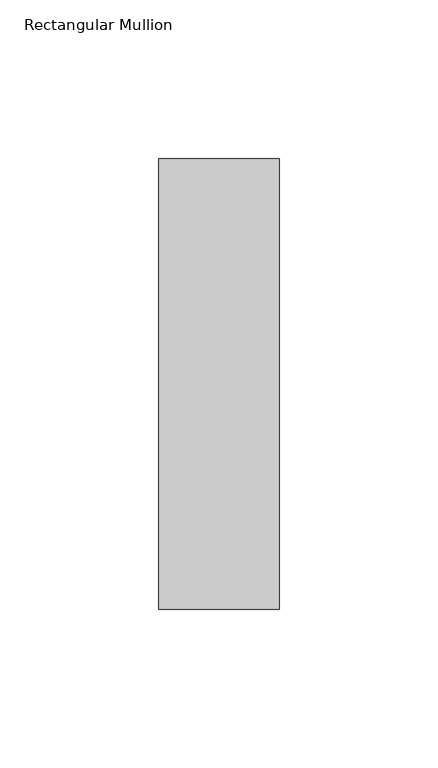
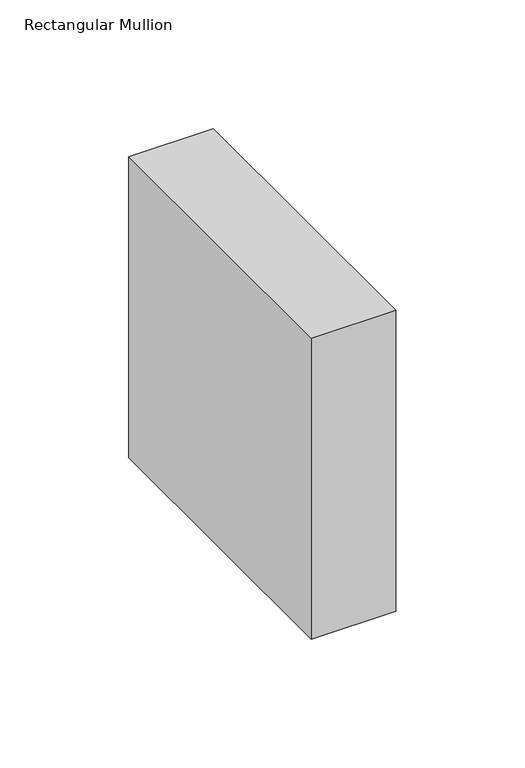
"""IFC4 building model written with IfcOpenShell, lengths in millimetres: member geometry, Rectangular Mullion : NLRS_21_CWM_hsb-regel 38x142_gen_rsf."""

from ifc_helpers import new_model, si_unit, frame, origin, place, context, project, spatial, polyline, outline, extrude, source, transform, mapped, element, save


def rectangular_mullion_f3eb0596(model_context):
    return source(origin(), model_context, "Body", "SweptSolid", [
        extrude(outline(polyline([(0.0, -71.0), (-38.0, -71.0), (-38.0, 71.0), (0.0, 71.0), (0.0, -71.0)])), frame((0.0, 0.0, -142.9999997), z_axis=(0.0, 0.0, 1.0), x_axis=(1.0, 0.0, 0.0)), (0.0, 0.0, 1.0), 142.9999997),
    ])


if __name__ == "__main__":
    model = new_model("IFC4")
    model_context = context("Model", 3, world=origin())
    ifc_project = project(units=[si_unit("LENGTHUNIT", "METRE", prefix="MILLI")], contexts=[model_context])
    site = spatial("IfcSite", under=ifc_project)
    building = spatial("IfcBuilding", under=site)
    placement = place(None, origin())
    rectangular_mullion_shape = rectangular_mullion_f3eb0596(model_context)
    element("IfcMember", 1, ObjectType="Rectangular Mullion : NLRS_21_CWM_hsb-regel 38x142_gen_rsf", at=placement, inside=building, context=model_context, shape_type="MappedRepresentation", body=[
        mapped(rectangular_mullion_shape, transform((0.0, 0.0, 0.0), x_axis=(1.0, 0.0, 0.0), y_axis=(0.0, 1.0, 0.0), z_axis=(0.0, 0.0, 1.0))),
    ])
    save(model, "model.ifc")

# Revit data of these elements
# Type "Rectangular Mullion : NLRS_21_CWM_hsb-regel 38x142_gen_rsf"
#   Export Type to IFC As = "IfcWall"
#   Type IfcGUID = "07M7mRoiH1CR8m_RSKIwpF"
#   Assembly Code = "21.10"
#   built-in parameter 1007322 = 0.465879 (stored number, unit not read)
#   built-in parameter 1007321 = 0.062336 (stored number, unit not read)
#   built-in parameter 1007320 = 0.062336 (stored number, unit not read)
# Element 1 (IfcMember, "Rectangular Mullion : NLRS_21_CWM_hsb-regel 38x142_gen_rsf")
#   Materials on its faces: "NLRS_i2_hout naaldhout vuren_gen_rsf"
# Materials
#   "NLRS_i2_hout naaldhout vuren_gen_rsf": class "I - Hout", colour RGB 234 199 147, transparency 0, Keynote = "i2", Manufacturer = "Revit Standards Foundation", URL = "www.revitstandards.org", Description = "hout vuren", Cost = 0
